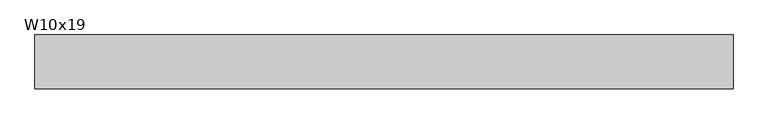
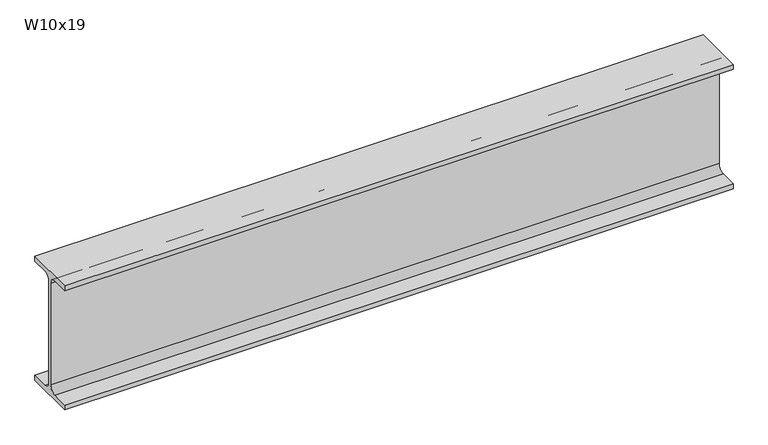
"""IFC4 building model written with IfcOpenShell, lengths in millimetres: beam geometry, RME W-Wide Flange : W10x19."""

import ifcopenshell
import ifcopenshell.guid

model = None  # the IFC model being written
_history = None  # IfcOwnerHistory: only IFC2X3 demands one
_inside = {}  # id of a spatial element -> (the spatial element, [elements in it])
_under = {}  # id of a project, library or spatial element -> (it, [spatial elements below it])
_declared = {}  # id of a project -> (the project, [libraries it declares])
_typed = {}  # id of a type object -> (the type object, [elements of that type])
_made_of = {}  # id of a material, layer set ... -> (it, [elements and type objects made of it])


def new_model(schema):
    """Start an empty IFC model of exactly this schema.

    Asked for "IFC4X3", IfcOpenShell would pick the latest addendum, in which some entities
    have other attributes; the version numbers below select the first issue.
    IFC2X3 requires an IfcOwnerHistory on every rooted entity: one is made here for all.
    """
    global model, _history
    if schema == "IFC4X3":
        model = ifcopenshell.file(schema_version=(4, 3, 0, 0))
    else:
        model = ifcopenshell.file(schema=schema)
    _inside.clear()
    _under.clear()
    _declared.clear()
    _typed.clear()
    _made_of.clear()
    _history = None
    if model.schema == "IFC2X3":
        org = make("IfcOrganization", Name="unknown")
        user = make(
            "IfcPersonAndOrganization",
            ThePerson=make("IfcPerson", FamilyName="unknown"),
            TheOrganization=org,
        )
        app = make(
            "IfcApplication",
            ApplicationDeveloper=org,
            Version="unknown",
            ApplicationFullName="unknown",
            ApplicationIdentifier="unknown",
        )
        _history = make(
            "IfcOwnerHistory",
            OwningUser=user,
            OwningApplication=app,
            ChangeAction="ADDED",
            CreationDate=0,
        )
    return model


def make(cls, **values):
    """One entity of the class cls with the attributes given. An attribute that is None is left unset."""
    return model.create_entity(
        cls, **{name: value for name, value in values.items() if value is not None}
    )


def rooted(cls, **values):
    """An entity with a GlobalId (a new one), such as an element, a storey or a relation."""
    return make(cls, GlobalId=ifcopenshell.guid.new(), OwnerHistory=_history, **values)


def si_unit(unit_type, name, prefix=None):
    """IfcSIUnit, for example si_unit("LENGTHUNIT", "METRE", prefix="MILLI")."""
    return make("IfcSIUnit", UnitType=unit_type, Prefix=prefix, Name=name)


def assignment(units):
    """IfcUnitAssignment: the units of a project."""
    return None if units is None else make("IfcUnitAssignment", Units=units)


def point(xyz):
    """IfcCartesianPoint."""
    return None if xyz is None else make("IfcCartesianPoint", Coordinates=xyz)


def direction(xyz):
    """IfcDirection."""
    return None if xyz is None else make("IfcDirection", DirectionRatios=xyz)


def frame(location, z_axis=None, x_axis=None):
    """IfcAxis2Placement3D, a coordinate frame: its origin and axes. An axis left out is left unset."""
    return make(
        "IfcAxis2Placement3D",
        Location=point(location),
        Axis=direction(z_axis),
        RefDirection=direction(x_axis),
    )


def frame_2d(location, x_axis=None):
    """IfcAxis2Placement2D, a coordinate frame in the plane: its origin and x axis."""
    return make(
        "IfcAxis2Placement2D", Location=point(location), RefDirection=direction(x_axis)
    )


def origin():
    """The frame at (0, 0, 0) with its axes left unset."""
    return frame((0.0, 0.0, 0.0))


def place(relative_to, where):
    """IfcLocalPlacement: puts the frame where relative to a parent placement (None: the world)."""
    return make(
        "IfcLocalPlacement", PlacementRelTo=relative_to, RelativePlacement=where
    )


def context(
    kind, dimensions, precision=None, world=None, true_north=None, identifier=None
):
    """IfcGeometricRepresentationContext, for example the 3D "Model" context."""
    return make(
        "IfcGeometricRepresentationContext",
        ContextIdentifier=identifier,
        ContextType=kind,
        CoordinateSpaceDimension=dimensions,
        Precision=precision,
        WorldCoordinateSystem=world,
        TrueNorth=true_north,
    )


def project(units=None, contexts=None):
    """IfcProject with its units and contexts."""
    return rooted(
        "IfcProject",
        Name="project",
        RepresentationContexts=contexts,
        UnitsInContext=assignment(units),
    )


def spatial(cls, under=None, at=None, **own):
    """A site, building, storey or space (cls), placed at a placement, below another one or the project."""
    s = rooted(cls, ObjectPlacement=at, **own)
    if under is not None:
        _under.setdefault(under.id(), (under, []))[1].append(s)
    return s


def polyline(points):
    """IfcPolyline through the points."""
    return make("IfcPolyline", Points=[point(p) for p in points])


def circle_curve(where, radius):
    """IfcCircle in the frame where."""
    return make("IfcCircle", Position=where, Radius=radius)


def trimmed(basis, trim1, trim2, sense, master):
    """IfcTrimmedCurve: the piece of a basis curve between two trims."""
    return make(
        "IfcTrimmedCurve",
        BasisCurve=basis,
        Trim1=trim1,
        Trim2=trim2,
        SenseAgreement=sense,
        MasterRepresentation=master,
    )


def segment(curve, same_sense, transition):
    """IfcCompositeCurveSegment."""
    return make(
        "IfcCompositeCurveSegment",
        Transition=transition,
        SameSense=same_sense,
        ParentCurve=curve,
    )


def composite_curve(segments, self_intersect=None):
    """IfcCompositeCurve: segments joined end to end."""
    return make("IfcCompositeCurve", Segments=segments, SelfIntersect=self_intersect)


def outline(outer, holes=None, kind="AREA"):
    """IfcArbitraryClosedProfileDef: a profile drawn as a closed curve; with holes, ...WithVoids."""
    if holes is None:
        return make("IfcArbitraryClosedProfileDef", ProfileType=kind, OuterCurve=outer)
    return make(
        "IfcArbitraryProfileDefWithVoids",
        ProfileType=kind,
        OuterCurve=outer,
        InnerCurves=holes,
    )


def extrude(swept, where, along, depth):
    """IfcExtrudedAreaSolid: the profile swept, set in the frame where, extruded along a direction by depth."""
    return make(
        "IfcExtrudedAreaSolid",
        SweptArea=swept,
        Position=where,
        ExtrudedDirection=direction(along),
        Depth=depth,
    )


def shape(context_of_items, identifier, shape_type, items):
    """IfcShapeRepresentation: the items that make up one representation, for example the "Body"."""
    return make(
        "IfcShapeRepresentation",
        ContextOfItems=context_of_items,
        RepresentationIdentifier=identifier,
        RepresentationType=shape_type,
        Items=items,
    )


def source(mapping_origin, context_of_items, identifier, shape_type, items):
    """IfcRepresentationMap: a shape defined once, which mapped items show again and again."""
    return make(
        "IfcRepresentationMap",
        MappingOrigin=mapping_origin,
        MappedRepresentation=shape(context_of_items, identifier, shape_type, items),
    )


def transform(
    local_origin,
    x_axis=None,
    y_axis=None,
    z_axis=None,
    scale=None,
    scale2=None,
    scale3=None,
    uniform=True,
):
    """IfcCartesianTransformationOperator3D, or its non-uniform kind. x_axis, y_axis, z_axis: its Axis1, 2, 3."""
    if uniform:
        return make(
            "IfcCartesianTransformationOperator3D",
            Axis1=direction(x_axis),
            Axis2=direction(y_axis),
            LocalOrigin=point(local_origin),
            Scale=scale,
            Axis3=direction(z_axis),
        )
    return make(
        "IfcCartesianTransformationOperator3DnonUniform",
        Axis1=direction(x_axis),
        Axis2=direction(y_axis),
        LocalOrigin=point(local_origin),
        Scale=scale,
        Axis3=direction(z_axis),
        Scale2=scale2,
        Scale3=scale3,
    )


def mapped(mapping_source, mapping_target):
    """IfcMappedItem: shows the shape of a source again, moved by a transform."""
    return make(
        "IfcMappedItem", MappingSource=mapping_source, MappingTarget=mapping_target
    )


def made_of(thing, what):
    """Note that an element or type object is made of a material, layer set ...; save() writes the relation."""
    if what is not None:
        _made_of.setdefault(what.id(), (what, []))[1].append(thing)
    return thing


def element(
    cls,
    number,
    at=None,
    inside=None,
    cuts=None,
    type_object=None,
    material=None,
    context=None,
    identifier="Body",
    shape_type=None,
    held_by="IfcProductDefinitionShape",
    body=None,
    shapes=None,
    **own,
):
    """One element of the class cls, such as IfcWall. Its Tag is "e" and its number.

    at: its placement. inside: the storey or other place that contains it. cuts: it is an
    opening in that element (IfcRelVoidsElement). A single representation is given by context,
    identifier, shape_type and body (its items); several are given by shapes. held_by: the class
    of the entity that holds the representations. save() writes the other relations.
    """
    e = rooted(cls, Tag="e%d" % number, ObjectPlacement=at, **own)
    if body is not None:
        shapes = [shape(context, identifier, shape_type, body)]
    if shapes is not None:
        e.Representation = make(held_by, Representations=shapes)
    if inside is not None:
        _inside.setdefault(inside.id(), (inside, []))[1].append(e)
    if cuts is not None:
        rooted(
            "IfcRelVoidsElement", RelatingBuildingElement=cuts, RelatedOpeningElement=e
        )
    if type_object is not None:
        _typed.setdefault(type_object.id(), (type_object, []))[1].append(e)
    return made_of(e, material)


def aggregate(whole, parts):
    """IfcRelAggregates: a whole, such as a stair, and the parts it consists of."""
    return rooted("IfcRelAggregates", RelatingObject=whole, RelatedObjects=parts)


def save(model, path):
    """Write the relations noted so far, then the file.

    IfcRelAggregates (storeys below a building ...), IfcRelContainedInSpatialStructure (elements
    in a storey), IfcRelDefinesByType, IfcRelAssociatesMaterial and IfcRelDeclares: one each for
    every whole, place, type object, material and project.
    """
    for whole, parts in _under.values():
        aggregate(whole, parts)
    for where, things in _inside.values():
        rooted(
            "IfcRelContainedInSpatialStructure",
            RelatedElements=things,
            RelatingStructure=where,
        )
    for kind, things in _typed.values():
        rooted("IfcRelDefinesByType", RelatedObjects=things, RelatingType=kind)
    for what, things in _made_of.values():
        rooted("IfcRelAssociatesMaterial", RelatedObjects=things, RelatingMaterial=what)
    for by, libraries in _declared.values():
        rooted("IfcRelDeclares", RelatingContext=by, RelatedDefinitions=libraries)
    model.write(path)


def w10x19_36e10caa(model_context):
    return source(origin(), model_context, "Body", "SweptSolid", [
        extrude(outline(composite_curve([segment(polyline([(51.054, -119.507), (51.054, -129.54), (-51.054, -129.54), (-51.054, -119.507), (-16.9545, -119.507)]), True, "CONTINUOUS"), segment(trimmed(circle_curve(frame_2d((-16.9545, -105.7275)), 13.7795), [point((-16.9545, -119.507))], [point((-3.175, -105.7275))], True, "CARTESIAN"), True, "CONTINUOUS"), segment(polyline([(-3.175, -105.7275), (-3.175, 105.7275)]), True, "CONTINUOUS"), segment(trimmed(circle_curve(frame_2d((-16.9545, 105.7275)), 13.7795), [point((-3.175, 105.7275))], [point((-16.9545, 119.507))], True, "CARTESIAN"), True, "CONTINUOUS"), segment(polyline([(-16.9545, 119.507), (-51.054, 119.507), (-51.054, 129.54), (51.054, 129.54), (51.054, 119.507), (16.9545, 119.507)]), True, "CONTINUOUS"), segment(trimmed(circle_curve(frame_2d((16.9545, 105.7275)), 13.7795), [point((16.9545, 119.507))], [point((3.175, 105.7275))], True, "CARTESIAN"), True, "CONTINUOUS"), segment(polyline([(3.175, 105.7275), (3.175, -105.7275)]), True, "CONTINUOUS"), segment(trimmed(circle_curve(frame_2d((16.9545, -105.7275)), 13.7795), [point((3.175, -105.7275))], [point((16.9545, -119.507))], True, "CARTESIAN"), True, "CONTINUOUS"), segment(polyline([(16.9545, -119.507), (51.054, -119.507)]), True, "CONTINUOUS")], self_intersect=False)), frame((-660.5388577, 0.0, 0.0), z_axis=(1.0, 0.0, 0.0), x_axis=(0.0, 1.0, 0.0)), (0.0, 0.0, 1.0), 1321.0777155),
    ])


if __name__ == "__main__":
    model = new_model("IFC4")
    model_context = context("Model", 3, world=origin())
    ifc_project = project(units=[si_unit("LENGTHUNIT", "METRE", prefix="MILLI")], contexts=[model_context])
    site = spatial("IfcSite", under=ifc_project)
    building = spatial("IfcBuilding", under=site)
    placement = place(None, origin())
    w10x19_shape = w10x19_36e10caa(model_context)
    element("IfcBeam", 1, ObjectType="RME W-Wide Flange : W10x19", at=placement, inside=building, context=model_context, shape_type="MappedRepresentation", body=[
        mapped(w10x19_shape, transform((0.0, 0.0, 0.0), x_axis=(1.0, 0.0, 0.0), y_axis=(0.0, 1.0, 0.0), z_axis=(0.0, 0.0, 1.0))),
    ])
    save(model, "model.ifc")

# Revit data of these elements
# Type "RME W-Wide Flange : W10x19"
#   WELD P [instance default] = ""
#   WELD LE [instance default] = ""
#   WELD D [instance default] = ""
#   TOP SECTION SIZE [instance default] = ""
#   TOP SECTION LENGTH [instance default] = ""
#   REMARKS [instance default] = ""
#   REINF TYPE [instance default] = ""
#   Nominal Size = "W24"
#   End Bearing Capacity [instance default] = ""
#   BOT SECTION SIZE [instance default] = ""
#   BOT SECTION LENGTH [instance default] = ""
#   Assembly Code = "B10"
#   W = 19
#   Start Extension Calculation [instance default] = 10' - 0"
#   Start Extension [instance default] = -0' - 0 1/2"
#   End Extension Calculation [instance default] = 10' - 0"
#   End Extension [instance default] = -0' - 0 1/2"
#   Length [instance default] = 5' - 0"
#   bf = 0' - 4.02"
#   d = 0' - 10.2"
#   k = 0' - 0 15/16"
#   k2 = 0' - 0.5425"
#   tf = 0' - 0.395"
#   tw = 0' - 0 1/4"
#   A = 0.0390278 SF
#   Structural Material [instance default] = Metal - Steel - ASTM A992
# Element 1 (IfcBeam, "RME W-Wide Flange : W10x19")
#   Length = 4' - 4.01093"
#   Materials on its faces: "Metal - Steel - ASTM A992"
# Materials
#   "Metal - Steel - ASTM A992": class "Metal", colour RGB 255 128 0, transparency 0
